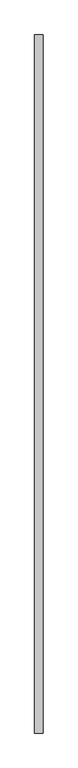
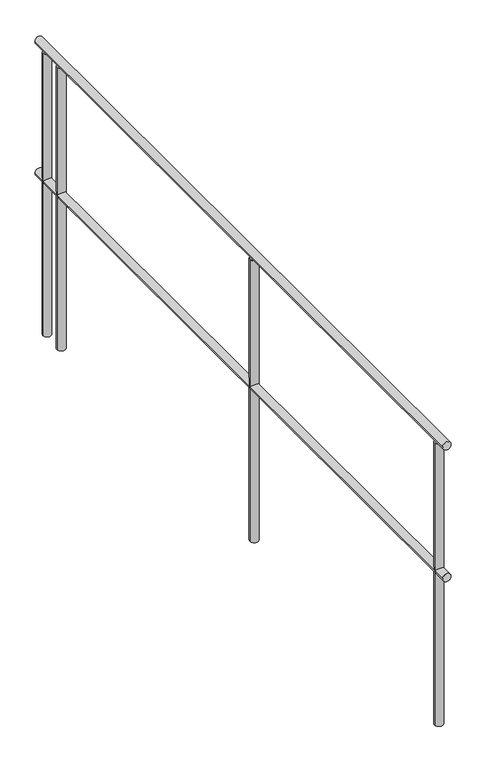
"""IFC4 building model written with IfcOpenShell, lengths in millimetres: railing geometry."""

from ifc_helpers import new_model, si_unit, point, frame, frame_2d, origin, place, context, project, spatial, circle_curve, trimmed, segment, composite_curve, outline, extrude, source, transform, mapped, element, save


def railing_0b3b75af(model_context):
    return source(origin(), model_context, "Body", "SweptSolid", [
        extrude(outline(composite_curve([segment(trimmed(circle_curve(frame_2d((885.0, 31537.1378478)), 15.0), [point((885.0, 31552.1378478))], [point((885.0, 31522.1378478))], False, "CARTESIAN"), True, "CONTINUOUS"), segment(trimmed(circle_curve(frame_2d((885.0, 31537.1378478)), 15.0), [point((885.0, 31522.1378478))], [point((885.0, 31552.1378478))], False, "CARTESIAN"), True, "CONTINUOUS")], self_intersect=False)), frame((0.0, 60949.5208589, 0.0), z_axis=(0.0, 1.0, 0.0), x_axis=(0.0, 0.0, 1.0)), (0.0, 0.0, 1.0), 2537.9),
        extrude(outline(composite_curve([segment(trimmed(circle_curve(frame_2d((1385.0, 31537.1378478)), 15.0), [point((1385.0, 31552.1378478))], [point((1385.0, 31522.1378478))], False, "CARTESIAN"), True, "CONTINUOUS"), segment(trimmed(circle_curve(frame_2d((1385.0, 31537.1378478)), 15.0), [point((1385.0, 31522.1378478))], [point((1385.0, 31552.1378478))], False, "CARTESIAN"), True, "CONTINUOUS")], self_intersect=False)), frame((0.0, 60949.5208589, 0.0), z_axis=(0.0, 1.0, 0.0), x_axis=(0.0, 0.0, 1.0)), (0.0, 0.0, 1.0), 2537.9),
        extrude(outline(composite_curve([segment(trimmed(circle_curve(frame_2d((31537.1378478, 63349.5208589)), 15.0), [point((31552.1378478, 63349.5208589))], [point((31522.1378478, 63349.5208589))], False, "CARTESIAN"), True, "CONTINUOUS"), segment(trimmed(circle_curve(frame_2d((31537.1378478, 63349.5208589)), 15.0), [point((31522.1378478, 63349.5208589))], [point((31552.1378478, 63349.5208589))], False, "CARTESIAN"), True, "CONTINUOUS")], self_intersect=False)), frame((0.0, 0.0, 300.0), z_axis=(0.0, 0.0, 1.0), x_axis=(1.0, 0.0, 0.0)), (0.0, 0.0, 1.0), 1070.0),
        extrude(outline(composite_curve([segment(trimmed(circle_curve(frame_2d((31537.1378478, 62149.5208589)), 15.0), [point((31552.1378478, 62149.5208589))], [point((31522.1378478, 62149.5208589))], False, "CARTESIAN"), True, "CONTINUOUS"), segment(trimmed(circle_curve(frame_2d((31537.1378478, 62149.5208589)), 15.0), [point((31522.1378478, 62149.5208589))], [point((31552.1378478, 62149.5208589))], False, "CARTESIAN"), True, "CONTINUOUS")], self_intersect=False)), frame((0.0, 0.0, 300.0), z_axis=(0.0, 0.0, 1.0), x_axis=(1.0, 0.0, 0.0)), (0.0, 0.0, 1.0), 1070.0),
        extrude(outline(composite_curve([segment(trimmed(circle_curve(frame_2d((31537.1378478, 63437.4208589)), 15.0), [point((31552.1378478, 63437.4208589))], [point((31522.1378478, 63437.4208589))], False, "CARTESIAN"), True, "CONTINUOUS"), segment(trimmed(circle_curve(frame_2d((31537.1378478, 63437.4208589)), 15.0), [point((31522.1378478, 63437.4208589))], [point((31552.1378478, 63437.4208589))], False, "CARTESIAN"), True, "CONTINUOUS")], self_intersect=False)), frame((0.0, 0.0, 300.0), z_axis=(0.0, 0.0, 1.0), x_axis=(1.0, 0.0, 0.0)), (0.0, 0.0, 1.0), 1070.0),
        extrude(outline(composite_curve([segment(trimmed(circle_curve(frame_2d((31537.1378478, 60999.5208589)), 15.0), [point((31552.1378478, 60999.5208589))], [point((31522.1378478, 60999.5208589))], False, "CARTESIAN"), True, "CONTINUOUS"), segment(trimmed(circle_curve(frame_2d((31537.1378478, 60999.5208589)), 15.0), [point((31522.1378478, 60999.5208589))], [point((31552.1378478, 60999.5208589))], False, "CARTESIAN"), True, "CONTINUOUS")], self_intersect=False)), frame((0.0, 0.0, 300.0), z_axis=(0.0, 0.0, 1.0), x_axis=(1.0, 0.0, 0.0)), (0.0, 0.0, 1.0), 1070.0),
    ])


if __name__ == "__main__":
    model = new_model("IFC4")
    model_context = context("Model", 3, world=origin())
    ifc_project = project(units=[si_unit("LENGTHUNIT", "METRE", prefix="MILLI")], contexts=[model_context])
    site = spatial("IfcSite", under=ifc_project)
    building = spatial("IfcBuilding", under=site)
    placement = place(None, origin())
    railing_shape = railing_0b3b75af(model_context)
    element("IfcRailing", 1, at=placement, inside=building, context=model_context, shape_type="MappedRepresentation", body=[
        mapped(railing_shape, transform((0.0, 0.0, 0.0), x_axis=(1.0, 0.0, 0.0), y_axis=(0.0, 1.0, 0.0), z_axis=(0.0, 0.0, 1.0))),
    ])
    save(model, "model.ifc")
